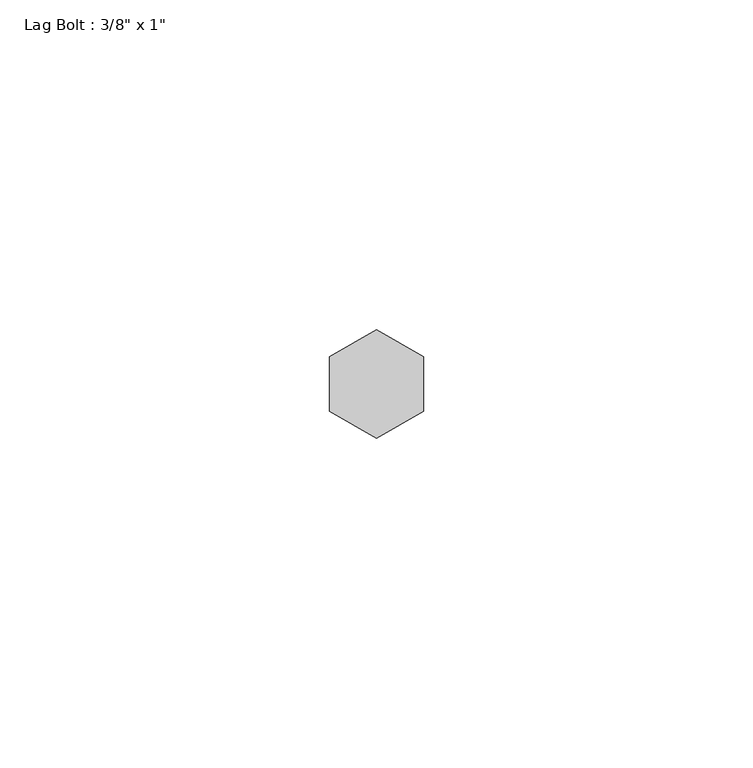
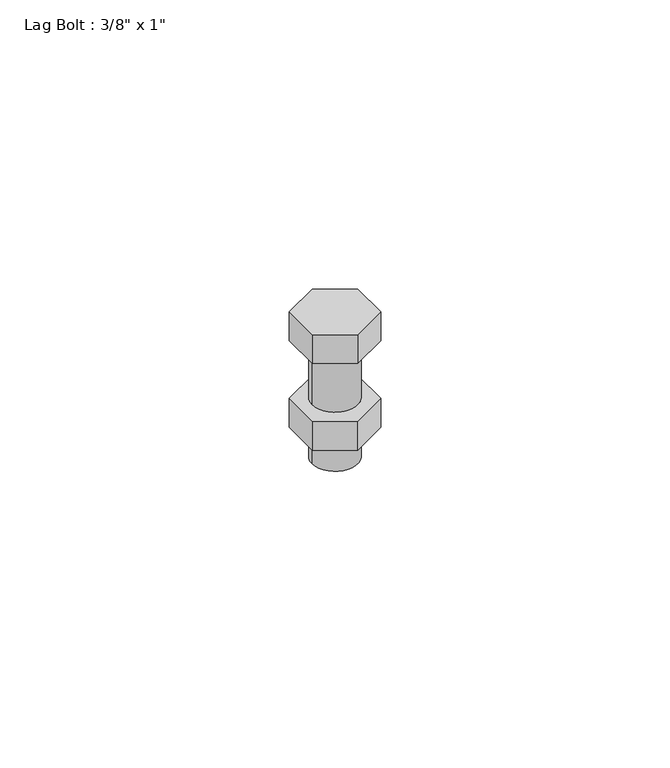
"""IFC4 building model written with IfcOpenShell, lengths in millimetres: proxy geometry."""

from ifc_helpers import new_model, si_unit, point, frame, origin, origin_with_axes, origin_2d, place, context, project, spatial, polyline, circle_curve, trimmed, segment, composite_curve, outline, extrude, source, transform, mapped, element, save


def proxy_a66d2f0e(model_context):
    return source(origin(), model_context, "Body", "SweptSolid", [
        extrude(outline(polyline([(-7.14375, -4.124446), (-7.14375, 4.124446), (0.0, 8.248892), (7.14375, 4.124446), (7.14375, -4.124446), (0.0, -8.248892), (-7.14375, -4.124446)])), frame((0.0, 0.0, -19.05), z_axis=(0.0, 0.0, 1.0), x_axis=(1.0, 0.0, 0.0)), (0.0, 0.0, 1.0), 6.35),
        extrude(outline(polyline([(-7.14375, 4.124446), (0.0, 8.248892), (7.14375, 4.124446), (7.14375, -4.124446), (0.0, -8.248892), (-7.14375, -4.124446), (-7.14375, 4.124446)])), origin_with_axes(), (0.0, 0.0, 1.0), 6.35),
        extrude(outline(composite_curve([segment(trimmed(circle_curve(origin_2d(), 4.7625), [point((-4.7625, 0.0))], [point((4.7625, 0.0))], False, "CARTESIAN"), True, "CONTINUOUS"), segment(trimmed(circle_curve(origin_2d(), 4.7625), [point((4.7625, 0.0))], [point((-4.7625, 0.0))], False, "CARTESIAN"), True, "CONTINUOUS")], self_intersect=False)), frame((0.0, 0.0, -25.4), z_axis=(0.0, 0.0, 1.0), x_axis=(1.0, 0.0, 0.0)), (0.0, 0.0, 1.0), 25.4),
    ])


if __name__ == "__main__":
    model = new_model("IFC4")
    model_context = context("Model", 3, world=origin())
    ifc_project = project(units=[si_unit("LENGTHUNIT", "METRE", prefix="MILLI")], contexts=[model_context])
    site = spatial("IfcSite", under=ifc_project)
    building = spatial("IfcBuilding", under=site)
    placement = place(None, origin())
    proxy_shape = proxy_a66d2f0e(model_context)
    element("IfcBuildingElementProxy", 1, Name="Lag Bolt : 3/8\" x 1\"", ObjectType="Lag Bolt : 3/8\" x 1\"", at=placement, inside=building, context=model_context, shape_type="MappedRepresentation", body=[
        mapped(proxy_shape, transform((0.0, 0.0, 0.0), x_axis=(1.0, 0.0, 0.0), y_axis=(0.0, 1.0, 0.0), z_axis=(0.0, 0.0, 1.0))),
    ])
    save(model, "model.ifc")

# Revit data of these elements
# Type "Lag Bolt : 3/8\" x 1\""
#   Thickness_of_Substrate [instance default] = 0' - 1"
#   Side = 0' - 0.3252"
#   Radius = 0' - 0 3/16"
#   Length = 0' - 1"
#   Head Size = 0' - 0 9/16"
#   Head Radius = 0' - 0 9/32"
#   Head Height = 0' - 0 1/4"
#   Diameter = 0' - 0 3/8"
#   Default Elevation = 4' - 0"
#   Nut_Visibility [instance default] = yes
#   Bolt Material (Size) [instance default] = STRUCTURAL BOLTS (PAINT TO MATCH STEEL FINISH)
# Element 1 (IfcBuildingElementProxy, "Lag Bolt : 3/8\" x 1\"")
#   Thickness_of_Substrate = 0' - 0 1/2"
#   Bolt Material (Size) = 3/8" X 1" GALV. BOLTS
#   Materials on its faces: "3/8\" X 1\" GALV. BOLTS", "STRUCTURAL BOLTS (PAINT TO MATCH STEEL FINISH)"
# Materials
#   "STRUCTURAL BOLTS (PAINT TO MATCH STEEL FINISH)": class "Generic", colour RGB 120 120 120, transparency 0, Cost = 0
#   "3/8\" X 1\" GALV. BOLTS": class "Generic", colour RGB 120 120 120, transparency 0, Cost = 0
